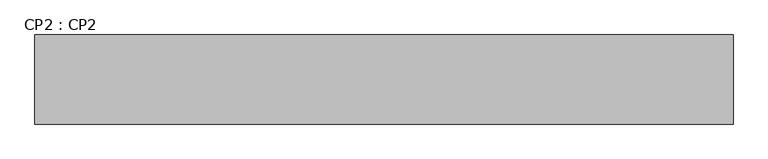
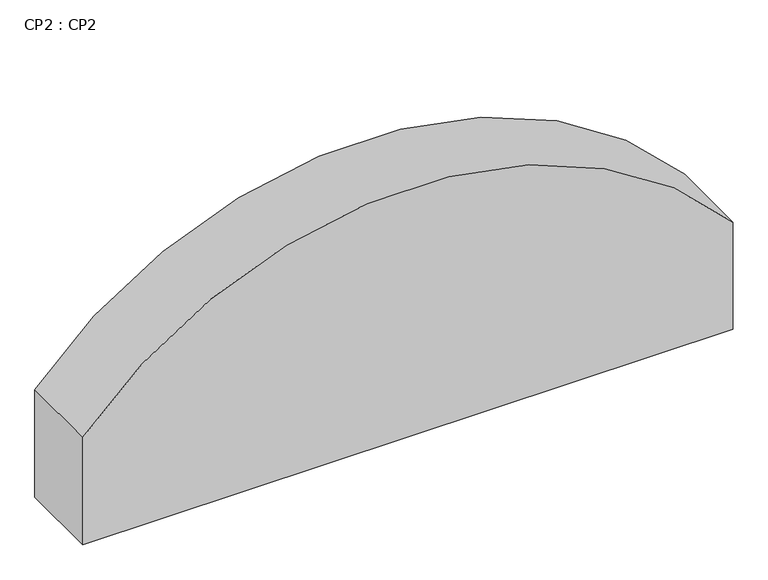
"""IFC4 building model written with IfcOpenShell, lengths in millimetres: beam geometry, CP2 : CP2."""

import ifcopenshell
import ifcopenshell.guid

model = None  # the IFC model being written
_history = None  # IfcOwnerHistory: only IFC2X3 demands one
_inside = {}  # id of a spatial element -> (the spatial element, [elements in it])
_under = {}  # id of a project, library or spatial element -> (it, [spatial elements below it])
_declared = {}  # id of a project -> (the project, [libraries it declares])
_typed = {}  # id of a type object -> (the type object, [elements of that type])
_made_of = {}  # id of a material, layer set ... -> (it, [elements and type objects made of it])


def new_model(schema):
    """Start an empty IFC model of exactly this schema.

    Asked for "IFC4X3", IfcOpenShell would pick the latest addendum, in which some entities
    have other attributes; the version numbers below select the first issue.
    IFC2X3 requires an IfcOwnerHistory on every rooted entity: one is made here for all.
    """
    global model, _history
    if schema == "IFC4X3":
        model = ifcopenshell.file(schema_version=(4, 3, 0, 0))
    else:
        model = ifcopenshell.file(schema=schema)
    _inside.clear()
    _under.clear()
    _declared.clear()
    _typed.clear()
    _made_of.clear()
    _history = None
    if model.schema == "IFC2X3":
        org = make("IfcOrganization", Name="unknown")
        user = make(
            "IfcPersonAndOrganization",
            ThePerson=make("IfcPerson", FamilyName="unknown"),
            TheOrganization=org,
        )
        app = make(
            "IfcApplication",
            ApplicationDeveloper=org,
            Version="unknown",
            ApplicationFullName="unknown",
            ApplicationIdentifier="unknown",
        )
        _history = make(
            "IfcOwnerHistory",
            OwningUser=user,
            OwningApplication=app,
            ChangeAction="ADDED",
            CreationDate=0,
        )
    return model


def make(cls, **values):
    """One entity of the class cls with the attributes given. An attribute that is None is left unset."""
    return model.create_entity(
        cls, **{name: value for name, value in values.items() if value is not None}
    )


def rooted(cls, **values):
    """An entity with a GlobalId (a new one), such as an element, a storey or a relation."""
    return make(cls, GlobalId=ifcopenshell.guid.new(), OwnerHistory=_history, **values)


def si_unit(unit_type, name, prefix=None):
    """IfcSIUnit, for example si_unit("LENGTHUNIT", "METRE", prefix="MILLI")."""
    return make("IfcSIUnit", UnitType=unit_type, Prefix=prefix, Name=name)


def assignment(units):
    """IfcUnitAssignment: the units of a project."""
    return None if units is None else make("IfcUnitAssignment", Units=units)


def point(xyz):
    """IfcCartesianPoint."""
    return None if xyz is None else make("IfcCartesianPoint", Coordinates=xyz)


def direction(xyz):
    """IfcDirection."""
    return None if xyz is None else make("IfcDirection", DirectionRatios=xyz)


def frame(location, z_axis=None, x_axis=None):
    """IfcAxis2Placement3D, a coordinate frame: its origin and axes. An axis left out is left unset."""
    return make(
        "IfcAxis2Placement3D",
        Location=point(location),
        Axis=direction(z_axis),
        RefDirection=direction(x_axis),
    )


def frame_2d(location, x_axis=None):
    """IfcAxis2Placement2D, a coordinate frame in the plane: its origin and x axis."""
    return make(
        "IfcAxis2Placement2D", Location=point(location), RefDirection=direction(x_axis)
    )


def origin():
    """The frame at (0, 0, 0) with its axes left unset."""
    return frame((0.0, 0.0, 0.0))


def place(relative_to, where):
    """IfcLocalPlacement: puts the frame where relative to a parent placement (None: the world)."""
    return make(
        "IfcLocalPlacement", PlacementRelTo=relative_to, RelativePlacement=where
    )


def context(
    kind, dimensions, precision=None, world=None, true_north=None, identifier=None
):
    """IfcGeometricRepresentationContext, for example the 3D "Model" context."""
    return make(
        "IfcGeometricRepresentationContext",
        ContextIdentifier=identifier,
        ContextType=kind,
        CoordinateSpaceDimension=dimensions,
        Precision=precision,
        WorldCoordinateSystem=world,
        TrueNorth=true_north,
    )


def project(units=None, contexts=None):
    """IfcProject with its units and contexts."""
    return rooted(
        "IfcProject",
        Name="project",
        RepresentationContexts=contexts,
        UnitsInContext=assignment(units),
    )


def spatial(cls, under=None, at=None, **own):
    """A site, building, storey or space (cls), placed at a placement, below another one or the project."""
    s = rooted(cls, ObjectPlacement=at, **own)
    if under is not None:
        _under.setdefault(under.id(), (under, []))[1].append(s)
    return s


def polyline(points):
    """IfcPolyline through the points."""
    return make("IfcPolyline", Points=[point(p) for p in points])


def circle_curve(where, radius):
    """IfcCircle in the frame where."""
    return make("IfcCircle", Position=where, Radius=radius)


def trimmed(basis, trim1, trim2, sense, master):
    """IfcTrimmedCurve: the piece of a basis curve between two trims."""
    return make(
        "IfcTrimmedCurve",
        BasisCurve=basis,
        Trim1=trim1,
        Trim2=trim2,
        SenseAgreement=sense,
        MasterRepresentation=master,
    )


def segment(curve, same_sense, transition):
    """IfcCompositeCurveSegment."""
    return make(
        "IfcCompositeCurveSegment",
        Transition=transition,
        SameSense=same_sense,
        ParentCurve=curve,
    )


def composite_curve(segments, self_intersect=None):
    """IfcCompositeCurve: segments joined end to end."""
    return make("IfcCompositeCurve", Segments=segments, SelfIntersect=self_intersect)


def outline(outer, holes=None, kind="AREA"):
    """IfcArbitraryClosedProfileDef: a profile drawn as a closed curve; with holes, ...WithVoids."""
    if holes is None:
        return make("IfcArbitraryClosedProfileDef", ProfileType=kind, OuterCurve=outer)
    return make(
        "IfcArbitraryProfileDefWithVoids",
        ProfileType=kind,
        OuterCurve=outer,
        InnerCurves=holes,
    )


def extrude(swept, where, along, depth):
    """IfcExtrudedAreaSolid: the profile swept, set in the frame where, extruded along a direction by depth."""
    return make(
        "IfcExtrudedAreaSolid",
        SweptArea=swept,
        Position=where,
        ExtrudedDirection=direction(along),
        Depth=depth,
    )


def shape(context_of_items, identifier, shape_type, items):
    """IfcShapeRepresentation: the items that make up one representation, for example the "Body"."""
    return make(
        "IfcShapeRepresentation",
        ContextOfItems=context_of_items,
        RepresentationIdentifier=identifier,
        RepresentationType=shape_type,
        Items=items,
    )


def source(mapping_origin, context_of_items, identifier, shape_type, items):
    """IfcRepresentationMap: a shape defined once, which mapped items show again and again."""
    return make(
        "IfcRepresentationMap",
        MappingOrigin=mapping_origin,
        MappedRepresentation=shape(context_of_items, identifier, shape_type, items),
    )


def transform(
    local_origin,
    x_axis=None,
    y_axis=None,
    z_axis=None,
    scale=None,
    scale2=None,
    scale3=None,
    uniform=True,
):
    """IfcCartesianTransformationOperator3D, or its non-uniform kind. x_axis, y_axis, z_axis: its Axis1, 2, 3."""
    if uniform:
        return make(
            "IfcCartesianTransformationOperator3D",
            Axis1=direction(x_axis),
            Axis2=direction(y_axis),
            LocalOrigin=point(local_origin),
            Scale=scale,
            Axis3=direction(z_axis),
        )
    return make(
        "IfcCartesianTransformationOperator3DnonUniform",
        Axis1=direction(x_axis),
        Axis2=direction(y_axis),
        LocalOrigin=point(local_origin),
        Scale=scale,
        Axis3=direction(z_axis),
        Scale2=scale2,
        Scale3=scale3,
    )


def mapped(mapping_source, mapping_target):
    """IfcMappedItem: shows the shape of a source again, moved by a transform."""
    return make(
        "IfcMappedItem", MappingSource=mapping_source, MappingTarget=mapping_target
    )


def made_of(thing, what):
    """Note that an element or type object is made of a material, layer set ...; save() writes the relation."""
    if what is not None:
        _made_of.setdefault(what.id(), (what, []))[1].append(thing)
    return thing


def element(
    cls,
    number,
    at=None,
    inside=None,
    cuts=None,
    type_object=None,
    material=None,
    context=None,
    identifier="Body",
    shape_type=None,
    held_by="IfcProductDefinitionShape",
    body=None,
    shapes=None,
    **own,
):
    """One element of the class cls, such as IfcWall. Its Tag is "e" and its number.

    at: its placement. inside: the storey or other place that contains it. cuts: it is an
    opening in that element (IfcRelVoidsElement). A single representation is given by context,
    identifier, shape_type and body (its items); several are given by shapes. held_by: the class
    of the entity that holds the representations. save() writes the other relations.
    """
    e = rooted(cls, Tag="e%d" % number, ObjectPlacement=at, **own)
    if body is not None:
        shapes = [shape(context, identifier, shape_type, body)]
    if shapes is not None:
        e.Representation = make(held_by, Representations=shapes)
    if inside is not None:
        _inside.setdefault(inside.id(), (inside, []))[1].append(e)
    if cuts is not None:
        rooted(
            "IfcRelVoidsElement", RelatingBuildingElement=cuts, RelatedOpeningElement=e
        )
    if type_object is not None:
        _typed.setdefault(type_object.id(), (type_object, []))[1].append(e)
    return made_of(e, material)


def aggregate(whole, parts):
    """IfcRelAggregates: a whole, such as a stair, and the parts it consists of."""
    return rooted("IfcRelAggregates", RelatingObject=whole, RelatedObjects=parts)


def save(model, path):
    """Write the relations noted so far, then the file.

    IfcRelAggregates (storeys below a building ...), IfcRelContainedInSpatialStructure (elements
    in a storey), IfcRelDefinesByType, IfcRelAssociatesMaterial and IfcRelDeclares: one each for
    every whole, place, type object, material and project.
    """
    for whole, parts in _under.values():
        aggregate(whole, parts)
    for where, things in _inside.values():
        rooted(
            "IfcRelContainedInSpatialStructure",
            RelatedElements=things,
            RelatingStructure=where,
        )
    for kind, things in _typed.values():
        rooted("IfcRelDefinesByType", RelatedObjects=things, RelatingType=kind)
    for what, things in _made_of.values():
        rooted("IfcRelAssociatesMaterial", RelatedObjects=things, RelatingMaterial=what)
    for by, libraries in _declared.values():
        rooted("IfcRelDeclares", RelatingContext=by, RelatedDefinitions=libraries)
    model.write(path)


def cp2_cp2_06c34e1b(model_context):
    return source(origin(), model_context, "Body", "SweptSolid", [
        extrude(outline(composite_curve([segment(trimmed(circle_curve(frame_2d((12603.8185575, 42833.2245513)), 3096.3668402), [point((14620.0, 45183.2245512))], [point((14620.0, 40483.2245513))], False, "CARTESIAN"), True, "CONTINUOUS"), segment(polyline([(14620.0, 40483.2245513), (13800.0, 40483.2245513), (13800.0, 45183.2245512), (14620.0, 45183.2245512)]), True, "CONTINUOUS")], self_intersect=False)), frame((0.0, -100.2551788, 0.0), z_axis=(0.0, 1.0, 0.0), x_axis=(0.0, 0.0, 1.0)), (0.0, 0.0, 1.0), 600.0),
    ])


if __name__ == "__main__":
    model = new_model("IFC4")
    model_context = context("Model", 3, world=origin())
    ifc_project = project(units=[si_unit("LENGTHUNIT", "METRE", prefix="MILLI")], contexts=[model_context])
    site = spatial("IfcSite", under=ifc_project)
    building = spatial("IfcBuilding", under=site)
    placement = place(None, origin())
    cp2_cp2_shape = cp2_cp2_06c34e1b(model_context)
    element("IfcBeam", 1, ObjectType="CP2 : CP2", at=placement, inside=building, context=model_context, shape_type="MappedRepresentation", body=[
        mapped(cp2_cp2_shape, transform((0.0, 0.0, 0.0), x_axis=(1.0, 0.0, 0.0), y_axis=(0.0, 1.0, 0.0), z_axis=(0.0, 0.0, 1.0))),
    ])
    save(model, "model.ifc")
